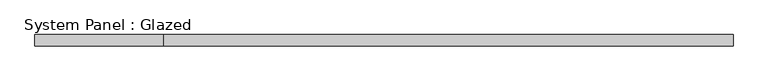
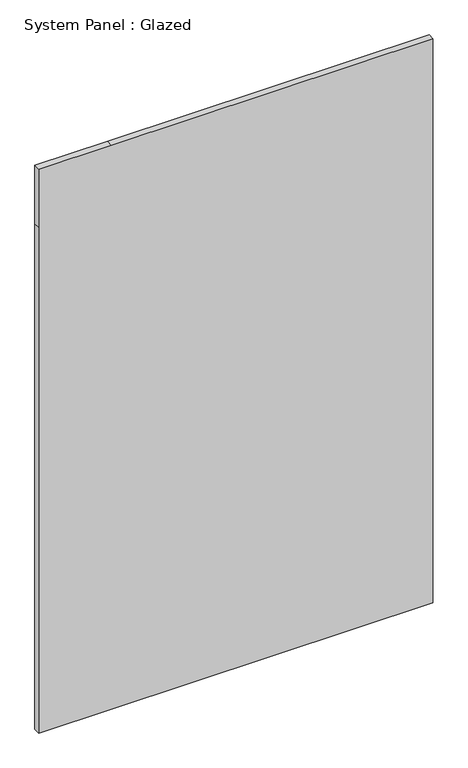
"""IFC4 building model written with IfcOpenShell, lengths in millimetres: plate geometry, System Panel : Glazed."""

from ifc_helpers import new_model, si_unit, frame, origin, place, context, project, spatial, polyline, outline, extrude, source, transform, mapped, element, save


def system_panel_glazed_00df446d(model_context):
    return source(origin(), model_context, "Body", "SweptSolid", [
        extrude(outline(polyline([(0.0, -774.7), (0.0, -488.95), (0.0, 774.7), (2101.85, 774.7), (2343.15, 774.7), (2343.15, -488.95), (2343.15, -774.7), (2101.85, -774.7), (0.0, -774.7)])), frame((0.0, 19.05, 0.0), z_axis=(0.0, 1.0, 0.0), x_axis=(0.0, 0.0, 1.0)), (0.0, 0.0, 1.0), 25.4),
    ])


if __name__ == "__main__":
    model = new_model("IFC4")
    model_context = context("Model", 3, world=origin())
    ifc_project = project(units=[si_unit("LENGTHUNIT", "METRE", prefix="MILLI")], contexts=[model_context])
    site = spatial("IfcSite", under=ifc_project)
    building = spatial("IfcBuilding", under=site)
    placement = place(None, origin())
    system_panel_glazed_shape = system_panel_glazed_00df446d(model_context)
    element("IfcPlate", 1, ObjectType="System Panel : Glazed", at=placement, inside=building, context=model_context, shape_type="MappedRepresentation", body=[
        mapped(system_panel_glazed_shape, transform((0.0, 0.0, 0.0), x_axis=(1.0, 0.0, 0.0), y_axis=(0.0, 1.0, 0.0), z_axis=(0.0, 0.0, 1.0))),
    ])
    save(model, "model.ifc")

# Revit data of these elements
# Element 1 (IfcPlate, "System Panel : Glazed")
#   Materials on its faces: "Glass"
# Materials
#   "Glass": class "Glass", colour RGB 0 128 192, transparency 0.75
